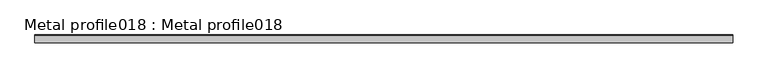
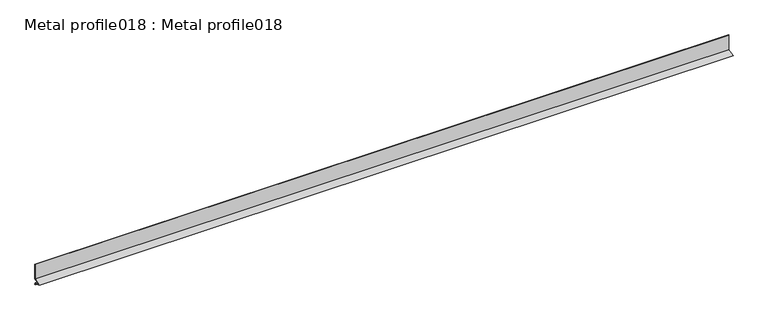
"""IFC4 building model written with IfcOpenShell, lengths in millimetres: proxy geometry, Metal profile018 : Metal profile018."""

from ifc_helpers import new_model, si_unit, frame, origin, place, context, project, spatial, polyline, outline, extrude, source, transform, mapped, element, save


def metal_profile018_metal_profile018_e56abe27(model_context):
    return source(origin(), model_context, "Body", "SweptSolid", [
        extrude(outline(polyline([(-4659.7667972, 36529.4059354), (-4661.0148598, 36529.1709038), (-4661.8381807, 36533.5428956), (-4681.9917972, 36540.0208437), (-4661.0367972, 36546.7563795), (-4661.0367972, 36590.8208437), (-4659.7667972, 36590.8208437), (-4659.7667972, 36545.8306002), (-4677.8415949, 36540.0208437), (-4660.7299923, 36534.5206858), (-4659.7667972, 36529.4059354)])), frame((12383.0178845, 0.0, 0.0), z_axis=(1.0, 0.0, 0.0), x_axis=(0.0, 1.0, 0.0)), (0.0, 0.0, 1.0), 2000.0),
    ])


if __name__ == "__main__":
    model = new_model("IFC4")
    model_context = context("Model", 3, world=origin())
    ifc_project = project(units=[si_unit("LENGTHUNIT", "METRE", prefix="MILLI")], contexts=[model_context])
    site = spatial("IfcSite", under=ifc_project)
    building = spatial("IfcBuilding", under=site)
    placement = place(None, origin())
    metal_profile018_metal_profile018_shape = metal_profile018_metal_profile018_e56abe27(model_context)
    element("IfcBuildingElementProxy", 1, Name="Metal profile018 : Metal profile018", ObjectType="Metal profile018 : Metal profile018", at=placement, inside=building, context=model_context, shape_type="MappedRepresentation", body=[
        mapped(metal_profile018_metal_profile018_shape, transform((0.0, 0.0, 0.0), x_axis=(1.0, 0.0, 0.0), y_axis=(0.0, 1.0, 0.0), z_axis=(0.0, 0.0, 1.0))),
    ])
    save(model, "model.ifc")

# Revit data of these elements
# Type "Metal profile018 : Metal profile018"
#   NameOverride = "Metal profile018"
# Element 1 (IfcBuildingElementProxy, "Metal profile018 : Metal profile018")
#   Materials on its faces: "16 GA. COPPER WEEP SCREED W/ MIN 3 1/2\" ATTACHMENT FLANGE - LAP UNDERLAYMENT OVER WEED SCREED"
# Materials
#   "16 GA. COPPER WEEP SCREED W/ MIN 3 1/2\" ATTACHMENT FLANGE - LAP UNDERLAYMENT OVER WEED SCREED": class "Unassigned", colour RGB 255 237 20, transparency 0
